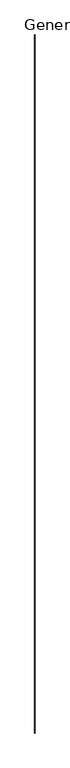
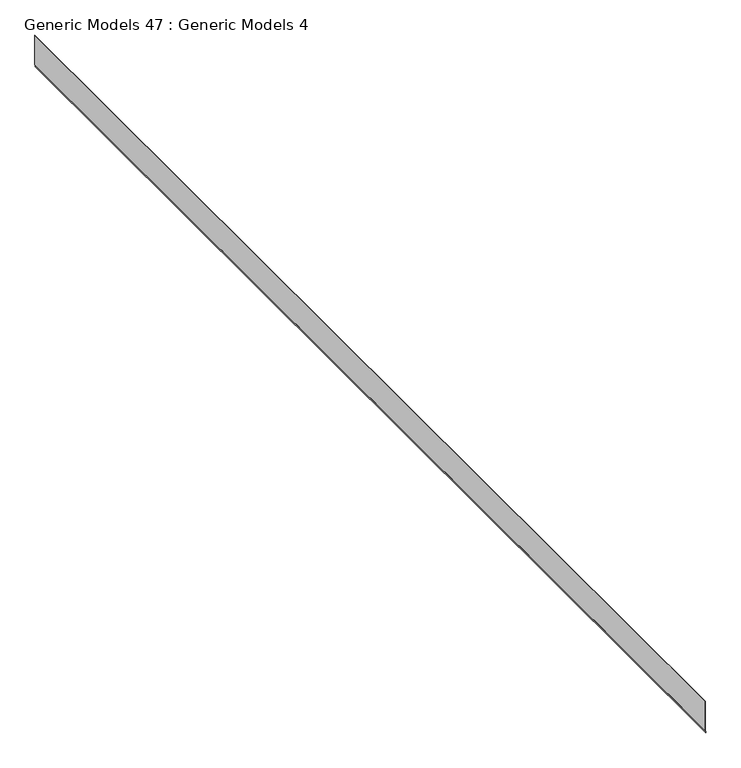
"""IFC4 building model written with IfcOpenShell, lengths in millimetres: proxy geometry, Generic Models 47 : Generic Models 4."""

from ifc_helpers import new_model, si_unit, frame, origin, place, context, project, spatial, polyline, outline, extrude, source, transform, mapped, element, save


def generic_models_47_generic_models_4_ffb730ac(model_context):
    return source(origin(), model_context, "Body", "SweptSolid", [
        extrude(outline(polyline([(126365.8983004, -9253.0996905), (126346.8643404, -9253.0996905), (126346.8643404, -9252.3059405), (126366.03826, -9252.3059405), (126377.5318209, -9256.4892545), (126752.096, -9256.4892545), (126752.096, -9257.2830045), (126377.3918613, -9257.2830045), (126365.8983004, -9253.0996905)])), frame((0.0, -6864.9230338, 0.0), z_axis=(0.0, 1.0, 0.0), x_axis=(0.0, 0.0, 1.0)), (0.0, 0.0, 1.0), 13919.2),
    ])


if __name__ == "__main__":
    model = new_model("IFC4")
    model_context = context("Model", 3, world=origin())
    ifc_project = project(units=[si_unit("LENGTHUNIT", "METRE", prefix="MILLI")], contexts=[model_context])
    site = spatial("IfcSite", under=ifc_project)
    building = spatial("IfcBuilding", under=site)
    placement = place(None, origin())
    generic_models_47_generic_models_4_shape = generic_models_47_generic_models_4_ffb730ac(model_context)
    element("IfcBuildingElementProxy", 1, Name="Generic Models 47 : Generic Models 4", ObjectType="Generic Models 47 : Generic Models 4", at=placement, inside=building, context=model_context, shape_type="MappedRepresentation", body=[
        mapped(generic_models_47_generic_models_4_shape, transform((0.0, 0.0, 0.0), x_axis=(1.0, 0.0, 0.0), y_axis=(0.0, 1.0, 0.0), z_axis=(0.0, 0.0, 1.0))),
    ])
    save(model, "model.ifc")

# Revit data of these elements
# Element 1 (IfcBuildingElementProxy, "Generic Models 47 : Generic Models 4")
#   Materials on its faces: "_(2) LAYERS NO. 30 ASTM D226 ASPHALT SATURATED ORGANIC FELT"
# Materials
#   "_(2) LAYERS NO. 30 ASTM D226 ASPHALT SATURATED ORGANIC FELT": class "Generic", colour RGB 67 154 161, transparency 0, Cost = 0
